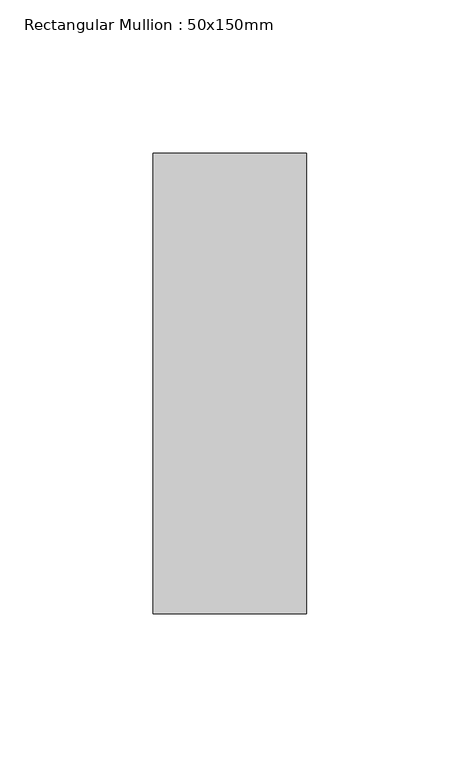
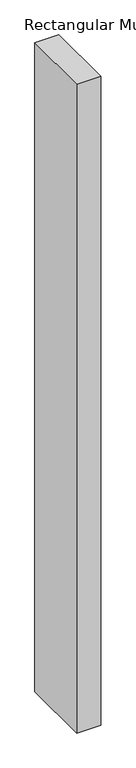
"""IFC4 building model written with IfcOpenShell, lengths in millimetres: member geometry, Rectangular Mullion : 50x150mm."""

from ifc_helpers import new_model, si_unit, frame, origin, place, context, project, spatial, polyline, outline, extrude, source, transform, mapped, element, save


def rectangular_mullion_50x150mm_1f4d75dd(model_context):
    return source(origin(), model_context, "Body", "SweptSolid", [
        extrude(outline(polyline([(25.0, 75.0), (25.0, -75.0), (-25.0, -75.0), (-25.0, 75.0), (25.0, 75.0)])), frame((0.0, 0.0, -1425.0), z_axis=(0.0, 0.0, 1.0), x_axis=(1.0, 0.0, 0.0)), (0.0, 0.0, 1.0), 1425.0),
    ])


if __name__ == "__main__":
    model = new_model("IFC4")
    model_context = context("Model", 3, world=origin())
    ifc_project = project(units=[si_unit("LENGTHUNIT", "METRE", prefix="MILLI")], contexts=[model_context])
    site = spatial("IfcSite", under=ifc_project)
    building = spatial("IfcBuilding", under=site)
    placement = place(None, origin())
    rectangular_mullion_50x150mm_shape = rectangular_mullion_50x150mm_1f4d75dd(model_context)
    element("IfcMember", 1, ObjectType="Rectangular Mullion : 50x150mm", at=placement, inside=building, context=model_context, shape_type="MappedRepresentation", body=[
        mapped(rectangular_mullion_50x150mm_shape, transform((0.0, 0.0, 0.0), x_axis=(1.0, 0.0, 0.0), y_axis=(0.0, 1.0, 0.0), z_axis=(0.0, 0.0, 1.0))),
    ])
    save(model, "model.ifc")

# Revit data of these elements
# Type "Rectangular Mullion : 50x150mm"
#   Keynote = "H11"
#   built-in parameter 1007304 = 0.492126 (stored number, unit not read)
#   built-in parameter 1007301 = 0.082021 (stored number, unit not read)
#   built-in parameter 1007300 = 0.082021 (stored number, unit not read)
# Element 1 (IfcMember, "Rectangular Mullion : 50x150mm")
#   Materials on its faces: "Aluminium"
# Materials
#   "Aluminium": class "Metal", colour RGB 247 247 247, transparency 0, Description = "Aluminium 6061", Cost = 0
